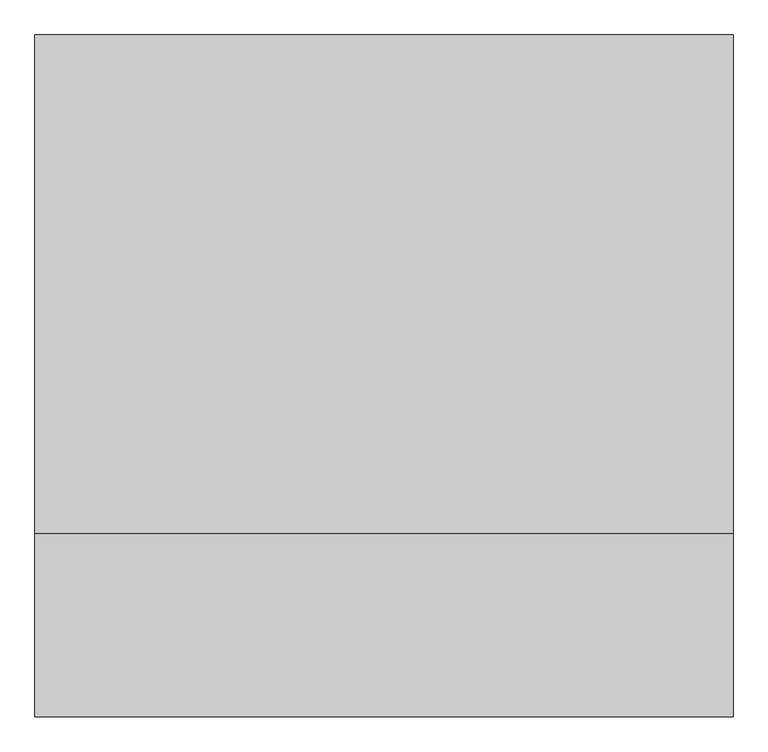
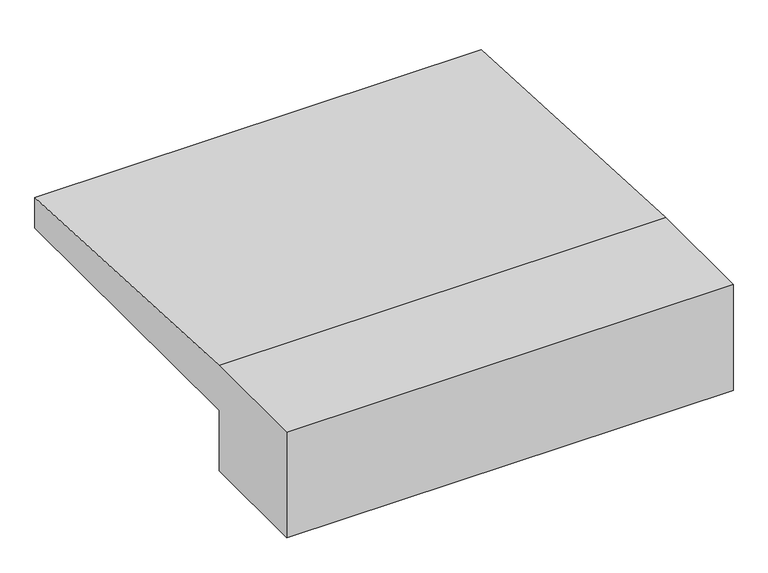
"""IFC4 building model written with IfcOpenShell, lengths in millimetres: plate geometry, 캐노피 : 캐노피."""

from ifc_helpers import new_model, si_unit, frame, origin, place, context, project, spatial, polyline, outline, extrude, source, transform, mapped, element, save


def plate_4d130048(model_context):
    return source(origin(), model_context, "Body", "SweptSolid", [
        extrude(outline(polyline([(-183.5, 800.0), (-183.5, 1150.0), (183.5, 1150.0), (1183.5, 1100.0), (1183.5, 1000.0), (183.5, 1000.0), (183.5, 800.0), (-183.5, 800.0)])), frame((-700.0, 0.0, 0.0), z_axis=(1.0, 0.0, 0.0), x_axis=(0.0, 1.0, 0.0)), (0.0, 0.0, 1.0), 1400.0),
    ])


if __name__ == "__main__":
    model = new_model("IFC4")
    model_context = context("Model", 3, world=origin())
    ifc_project = project(units=[si_unit("LENGTHUNIT", "METRE", prefix="MILLI")], contexts=[model_context])
    site = spatial("IfcSite", under=ifc_project)
    building = spatial("IfcBuilding", under=site)
    placement = place(None, origin())
    plate_shape = plate_4d130048(model_context)
    element("IfcPlate", 1, ObjectType="캐노피 : 캐노피", at=placement, inside=building, context=model_context, shape_type="MappedRepresentation", body=[
        mapped(plate_shape, transform((0.0, 0.0, 0.0), x_axis=(1.0, 0.0, 0.0), y_axis=(0.0, 1.0, 0.0), z_axis=(0.0, 0.0, 1.0))),
    ])
    save(model, "model.ifc")

# Revit data of these elements
# Type "캐노피 : 캐노피"
#   Type Mark = "203"
#   Width = 1400 mm
#   Height = 350 mm
#   돌출길이 = 1000 mm
#   Default Sill Height = 800 mm
#   Wall Closure = (empty or 0)
